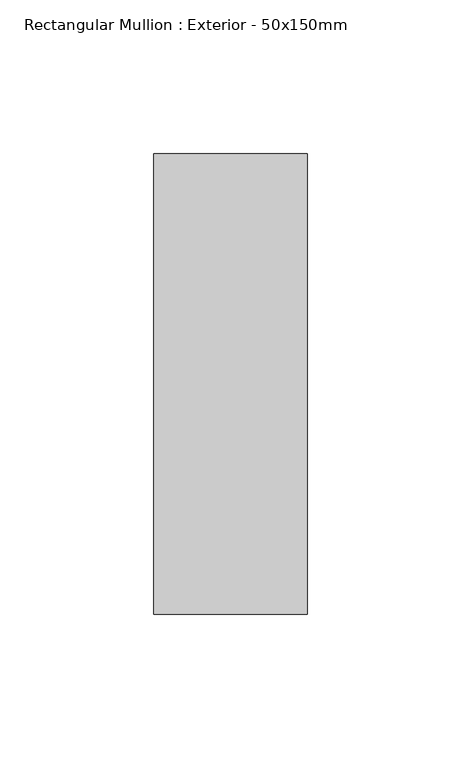
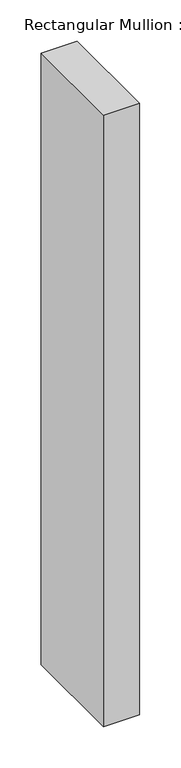
"""IFC4 building model written with IfcOpenShell, lengths in millimetres: member geometry, Rectangular Mullion : Exterior - 50x150mm."""

from ifc_helpers import new_model, si_unit, frame, origin, place, context, project, spatial, polyline, outline, extrude, source, transform, mapped, element, save


def rectangular_mullion_exterior_50x150mm_23692360(model_context):
    return source(origin(), model_context, "Body", "SweptSolid", [
        extrude(outline(polyline([(25.0, 0.0), (25.0, -150.0), (-25.0, -150.0), (-25.0, 0.0), (25.0, 0.0)])), frame((0.0, 0.0, -900.0), z_axis=(0.0, 0.0, 1.0), x_axis=(1.0, 0.0, 0.0)), (0.0, 0.0, 1.0), 900.0),
    ])


if __name__ == "__main__":
    model = new_model("IFC4")
    model_context = context("Model", 3, world=origin())
    ifc_project = project(units=[si_unit("LENGTHUNIT", "METRE", prefix="MILLI")], contexts=[model_context])
    site = spatial("IfcSite", under=ifc_project)
    building = spatial("IfcBuilding", under=site)
    placement = place(None, origin())
    rectangular_mullion_exterior_50x150mm_shape = rectangular_mullion_exterior_50x150mm_23692360(model_context)
    element("IfcMember", 1, ObjectType="Rectangular Mullion : Exterior - 50x150mm", at=placement, inside=building, context=model_context, shape_type="MappedRepresentation", body=[
        mapped(rectangular_mullion_exterior_50x150mm_shape, transform((0.0, 0.0, 0.0), x_axis=(1.0, 0.0, 0.0), y_axis=(0.0, 1.0, 0.0), z_axis=(0.0, 0.0, 1.0))),
    ])
    save(model, "model.ifc")

# Revit data of these elements
# Type "Rectangular Mullion : Exterior - 50x150mm"
#   built-in parameter 1007351 = -0.246063 (stored number, unit not read)
#   built-in parameter 1007304 = 0.492126 (stored number, unit not read)
#   built-in parameter 1007301 = 0.082021 (stored number, unit not read)
#   built-in parameter 1007300 = 0.082021 (stored number, unit not read)
# Element 1 (IfcMember, "Rectangular Mullion : Exterior - 50x150mm")
#   Materials on its faces: "Default Frame/Mullion (Interior/Exterior)"
# Materials
#   "Default Frame/Mullion (Interior/Exterior)": class "Generic", colour RGB 205 205 205, transparency 0, Description = "Udefineret karm/ramme materiale", Cost = 0
